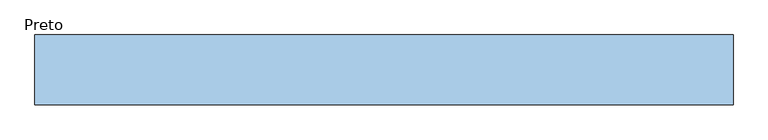
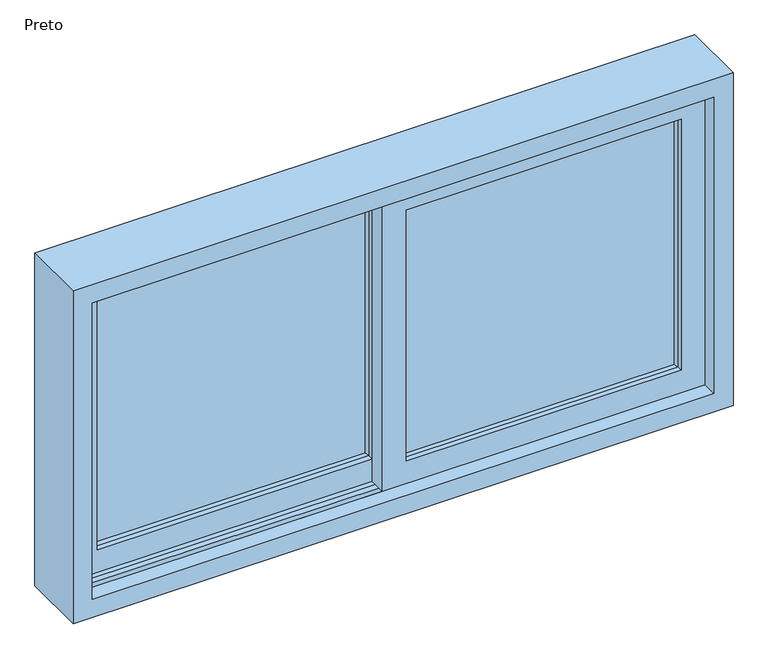
"""IFC4 building model written with IfcOpenShell, lengths in millimetres: window geometry, Blks_Cons Weiku_Janela de Correr 02 Folhas : Preto."""

from ifc_helpers import new_model, si_unit, frame, origin, place, context, project, spatial, polyline, outline, extrude, faceted_brep, source, transform, mapped, element, save


def preto_2c286093(model_context):
    return source(origin(), model_context, "Body", "SolidModel", [
        faceted_brep([(27.0, -13.0, 898.0), (27.0, -18.0, 898.0), (27.0, -18.0, 1502.0), (27.0, -13.0, 1502.0), (32.0, -18.0, 903.0), (32.0, -18.0, 1497.0), (652.0, -18.0, 1502.0), (652.0, -13.0, 1502.0), (647.0, -18.0, 1497.0), (652.0, -18.0, 898.0), (652.0, -13.0, 898.0), (647.0, -18.0, 903.0)], [[[0, 1, 2, 3]], [[4, 0, 3, 5]], [[3, 2, 6, 7]], [[5, 3, 7, 8]], [[7, 6, 9, 10]], [[8, 7, 10, 11]], [[1, 9, 6, 2], [5, 8, 11, 4]], [[10, 9, 1, 0]], [[11, 10, 0, 4]]]),
        faceted_brep([(652.0, -27.0, 898.0), (652.0, -22.0, 898.0), (652.0, -22.0, 1502.0), (652.0, -27.0, 1502.0), (27.0, -22.0, 1502.0), (27.0, -27.0, 1502.0), (27.0, -22.0, 898.0), (27.0, -27.0, 898.0), (647.0, -22.0, 1497.0), (32.0, -22.0, 1497.0), (32.0, -22.0, 903.0), (647.0, -22.0, 903.0)], [[[0, 1, 2, 3]], [[3, 2, 4, 5]], [[5, 4, 6, 7]], [[1, 6, 4, 2], [8, 9, 10, 11]], [[7, 6, 1, 0]], [[11, 0, 3, 8]], [[8, 3, 5, 9]], [[9, 5, 7, 10]], [[10, 7, 0, 11]]]),
        extrude(outline(polyline([(652.0, -22.0), (27.0, -22.0), (27.0, -18.0), (652.0, -18.0), (652.0, -22.0)])), frame((0.0, 0.0, 898.0), z_axis=(0.0, 0.0, 1.0), x_axis=(1.0, 0.0, 0.0)), (0.0, 0.0, 1.0), 604.0),
        extrude(outline(polyline([(844.0, 706.0), (1556.0, 706.0), (1556.0, -27.0), (844.0, -27.0), (844.0, 706.0)]), holes=[polyline([(1502.0, 27.0), (1502.0, 652.0), (898.0, 652.0), (898.0, 27.0), (1502.0, 27.0)])]), frame((0.0, -40.0, 0.0), z_axis=(0.0, 1.0, 0.0), x_axis=(0.0, 0.0, 1.0)), (0.0, 0.0, 1.0), 40.0),
        faceted_brep([(-652.0, 27.0, 898.0), (-652.0, 22.0, 898.0), (-652.0, 22.0, 1502.0), (-652.0, 27.0, 1502.0), (-647.0, 22.0, 903.0), (-647.0, 22.0, 1497.0), (-27.0, 22.0, 1502.0), (-27.0, 27.0, 1502.0), (-32.0, 22.0, 1497.0), (-27.0, 22.0, 898.0), (-27.0, 27.0, 898.0), (-32.0, 22.0, 903.0)], [[[0, 1, 2, 3]], [[4, 0, 3, 5]], [[3, 2, 6, 7]], [[5, 3, 7, 8]], [[7, 6, 9, 10]], [[8, 7, 10, 11]], [[1, 9, 6, 2], [5, 8, 11, 4]], [[10, 9, 1, 0]], [[11, 10, 0, 4]]]),
        faceted_brep([(-27.0, 13.0, 898.0), (-27.0, 18.0, 898.0), (-27.0, 18.0, 1502.0), (-27.0, 13.0, 1502.0), (-652.0, 18.0, 1502.0), (-652.0, 13.0, 1502.0), (-652.0, 18.0, 898.0), (-652.0, 13.0, 898.0), (-32.0, 18.0, 1497.0), (-647.0, 18.0, 1497.0), (-647.0, 18.0, 903.0), (-32.0, 18.0, 903.0)], [[[0, 1, 2, 3]], [[3, 2, 4, 5]], [[5, 4, 6, 7]], [[1, 6, 4, 2], [8, 9, 10, 11]], [[7, 6, 1, 0]], [[11, 0, 3, 8]], [[8, 3, 5, 9]], [[9, 5, 7, 10]], [[10, 7, 0, 11]]]),
        extrude(outline(polyline([(-27.0, 18.0), (-652.0, 18.0), (-652.0, 22.0), (-27.0, 22.0), (-27.0, 18.0)])), frame((0.0, 0.0, 898.0), z_axis=(0.0, 0.0, 1.0), x_axis=(1.0, 0.0, 0.0)), (0.0, 0.0, 1.0), 604.0),
        extrude(outline(polyline([(844.0, 27.0), (1556.0, 27.0), (1556.0, -706.0), (844.0, -706.0), (844.0, 27.0)]), holes=[polyline([(1502.0, -652.0), (1502.0, -27.0), (898.0, -27.0), (898.0, -652.0), (1502.0, -652.0)])]), frame((0.0, 0.0, 0.0), z_axis=(0.0, 1.0, 0.0), x_axis=(0.0, 0.0, 1.0)), (0.0, 0.0, 1.0), 40.0),
        faceted_brep([(706.0, 75.0, 844.0), (-706.0, 75.0, 844.0), (-706.0, 40.0, 844.0), (706.0, 40.0, 844.0), (-706.0, -75.0, 844.0), (706.0, -75.0, 844.0), (706.0, -40.0, 844.0), (-706.0, -40.0, 844.0), (-706.0, -13.0, 844.0), (-706.0, -27.0, 844.0), (706.0, -27.0, 844.0), (706.0, -13.0, 844.0), (-706.0, 27.0, 844.0), (-706.0, 13.0, 844.0), (706.0, 13.0, 844.0), (706.0, 27.0, 844.0), (750.0, 75.0, 800.0), (-750.0, 75.0, 800.0), (-750.0, 75.0, 1600.0), (750.0, 75.0, 1600.0), (706.0, 75.0, 1556.0), (-706.0, 75.0, 1556.0), (-706.0, 40.0, 1556.0), (-706.0, 40.0, 1566.0), (-706.0, 27.0, 1566.0), (-706.0, 27.0, 1556.0), (-706.0, 13.0, 1556.0), (-706.0, 13.0, 1566.0), (-706.0, -13.0, 1566.0), (-706.0, -13.0, 1556.0), (-706.0, -27.0, 1556.0), (-706.0, -27.0, 1566.0), (-706.0, -40.0, 1566.0), (-706.0, -40.0, 1556.0), (-706.0, -75.0, 1556.0), (-706.0, -40.0, 834.0), (-706.0, -27.0, 834.0), (-706.0, -13.0, 834.0), (-706.0, 13.0, 834.0), (-706.0, 27.0, 834.0), (-706.0, 40.0, 834.0), (706.0, 40.0, 834.0), (706.0, 27.0, 834.0), (706.0, 13.0, 834.0), (706.0, -13.0, 834.0), (706.0, -27.0, 834.0), (706.0, -40.0, 834.0), (706.0, -75.0, 1556.0), (706.0, -40.0, 1556.0), (706.0, -40.0, 1566.0), (706.0, -27.0, 1566.0), (706.0, -27.0, 1556.0), (706.0, -13.0, 1556.0), (706.0, -13.0, 1566.0), (706.0, 13.0, 1566.0), (706.0, 13.0, 1556.0), (706.0, 27.0, 1556.0), (706.0, 27.0, 1566.0), (706.0, 40.0, 1566.0), (706.0, 40.0, 1556.0), (-750.0, -75.0, 800.0), (750.0, -75.0, 800.0), (750.0, -75.0, 1600.0), (-750.0, -75.0, 1600.0)], [[[0, 1, 2, 3]], [[4, 5, 6, 7]], [[8, 9, 10, 11]], [[12, 13, 14, 15]], [[16, 17, 18, 19], [1, 0, 20, 21]], [[1, 21, 22, 23, 24, 25, 26, 27, 28, 29, 30, 31, 32, 33, 34, 4, 7, 35, 36, 9, 8, 37, 38, 13, 12, 39, 40, 2]], [[40, 41, 3, 2]], [[20, 0, 3, 41, 42, 15, 14, 43, 44, 11, 10, 45, 46, 6, 5, 47, 48, 49, 50, 51, 52, 53, 54, 55, 56, 57, 58, 59]], [[60, 61, 62, 63], [5, 4, 34, 47]], [[46, 35, 7, 6]], [[45, 10, 9, 36]], [[11, 44, 37, 8]], [[43, 14, 13, 38]], [[15, 42, 39, 12]], [[61, 16, 19, 62]], [[16, 61, 60, 17]], [[17, 60, 63, 18]], [[46, 45, 36, 35]], [[44, 43, 38, 37]], [[42, 41, 40, 39]], [[26, 25, 56, 55]], [[30, 29, 52, 51]], [[21, 20, 59, 22]], [[47, 34, 33, 48]], [[18, 63, 62, 19]], [[55, 54, 27, 26]], [[54, 53, 28, 27]], [[53, 52, 29, 28]], [[51, 50, 31, 30]], [[50, 49, 32, 31]], [[32, 49, 48, 33]], [[58, 23, 22, 59]], [[58, 57, 24, 23]], [[57, 56, 25, 24]]]),
    ])


if __name__ == "__main__":
    model = new_model("IFC4")
    model_context = context("Model", 3, world=origin())
    ifc_project = project(units=[si_unit("LENGTHUNIT", "METRE", prefix="MILLI")], contexts=[model_context])
    site = spatial("IfcSite", under=ifc_project)
    building = spatial("IfcBuilding", under=site)
    placement = place(None, origin())
    preto_shape = preto_2c286093(model_context)
    element("IfcWindow", 1, ObjectType="Blks_Cons Weiku_Janela de Correr 02 Folhas : Preto", at=placement, inside=building, context=model_context, shape_type="MappedRepresentation", body=[
        mapped(preto_shape, transform((0.0, 0.0, 0.0), x_axis=(1.0, 0.0, 0.0), y_axis=(0.0, 1.0, 0.0), z_axis=(0.0, 0.0, 1.0))),
    ])
    save(model, "model.ifc")

# Revit data of these elements
# Type "Blks_Cons Weiku_Janela de Correr 02 Folhas : Preto"
#   Type Mark = "J26"
#   Type Comments = "Janela de Correr 02 Folhas"
#   Manufacturer = "Weiku"
#   Created By / Criado Por / Creado por = "Blocks"
#   Author URL = "https://BlocksRvt.com/"
#   Author Contact = "info@blocksrvt.com"
#   Assembly Code = "Cons"
#   c [instance default] = 250 mm
#   b [instance default] = 912 mm
#   a [instance default] = 983 mm
#   Rough Width [instance default] = 2000 mm
#   Width [instance default] = 1912 mm
#   Espessura Folha [instance default] = 40 mm
#   Rough Height [instance default] = 1000 mm
#   Height [instance default] = 912 mm
#   Abertura Janela Equerda [instance default] = 0 mm
#   Abertura Janela Direita [instance default] = 0 mm
#   Vidro = .vidro_growarq
#   Vedação = Blks - Rubber - Black
#   Janela = Blks - Plastic - Black - Glazed
#   Wall Closure = (empty or 0)
# Element 1 (IfcWindow, "Blks_Cons Weiku_Janela de Correr 02 Folhas : Preto")
#   b = 712 mm
#   a = 733 mm
#   Rough Width = 1500 mm
#   Width = 1412 mm
#   Rough Height = 800 mm
#   Height = 712 mm
#   Materials on its faces: "Blks - Plastic - Black - Glazed", "Blks - Rubber - Black", ".vidro_growarq"
# Materials
#   ".vidro_growarq": class "Vidro", colour RGB 200 215 215, transparency 0.6, Description = "Vidroverde", Cost = 0
#   "Blks - Rubber - Black": class "Paint/Coating", colour RGB 38 38 38, transparency 0, Cost = 0
#   "Blks - Plastic - Black - Glazed": class "Plastic", colour RGB 25 25 25, transparency 0, Cost = 0
